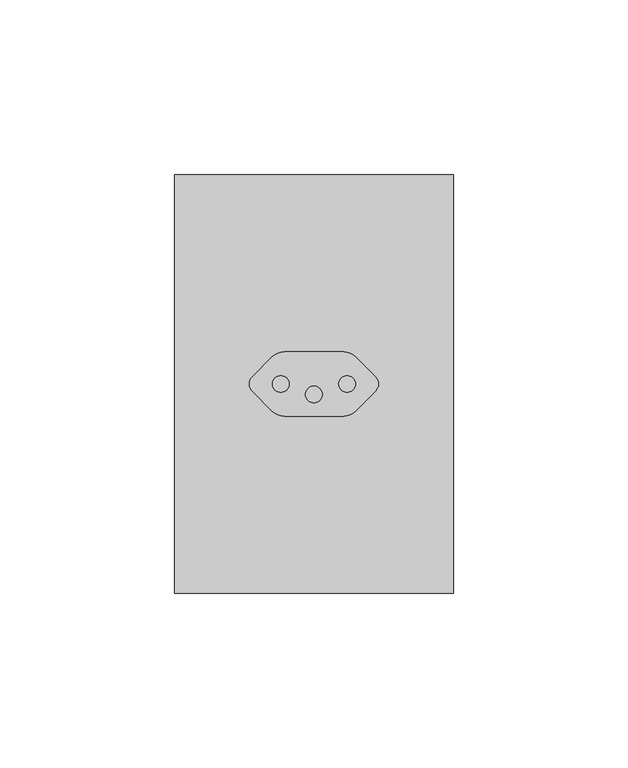
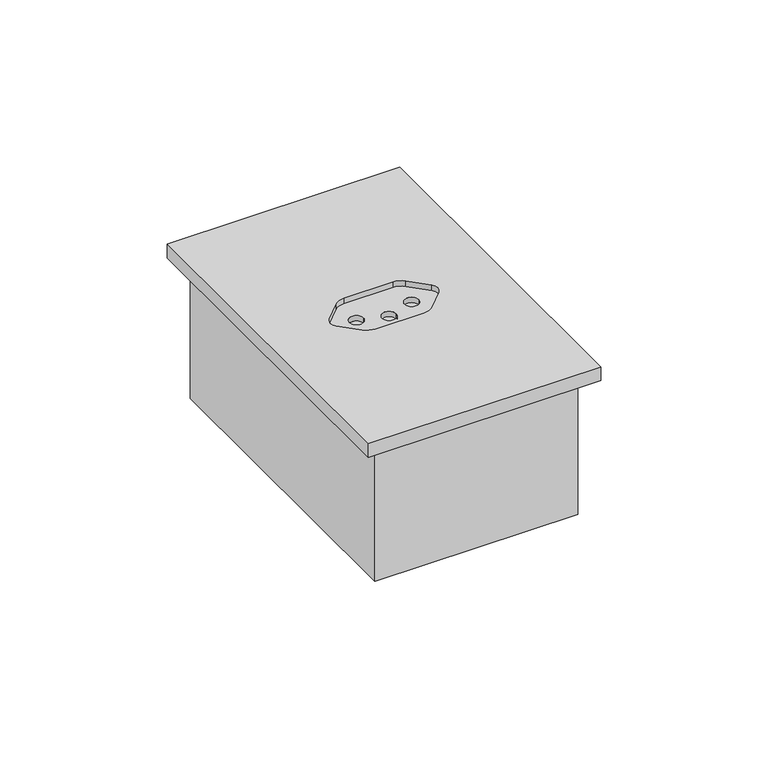
"""IFC4 building model written with IfcOpenShell, lengths in millimetres: proxy geometry, CAIXA VERTICE V7 : Tomada 20A 1s."""

from ifc_helpers import new_model, si_unit, frame, origin, place, context, project, spatial, polyline, circle_curve, faceted_brep, source, transform, mapped, element, save
from ifc_brep_helpers import plane_surface, revolved_surface, advanced_brep


def electrical_fixtures_8ee4f71d(model_context):
    return source(origin(), model_context, "Body", "SolidModel", [
        faceted_brep([(33.0, -2147.0, -48.0), (-33.0, -2147.0, -48.0), (-33.0, -2253.0, -48.0), (33.0, -2253.0, -48.0), (35.0, -2255.0, -50.0), (-35.0, -2255.0, -50.0), (-35.0, -2145.0, -50.0), (35.0, -2145.0, -50.0), (35.0, -2255.0, 0.0), (-35.0, -2255.0, 0.0), (-35.0, -2145.0, 0.0), (35.0, -2145.0, 0.0), (33.0, -2253.0, 0.0), (-33.0, -2253.0, 0.0), (-33.0, -2147.0, 0.0), (33.0, -2147.0, 0.0)], [[[0, 1, 2, 3]], [[4, 5, 6, 7]], [[4, 8, 9, 5]], [[9, 10, 6, 5]], [[10, 11, 7, 6]], [[11, 8, 4, 7]], [[8, 11, 10, 9], [12, 13, 14, 15]], [[15, 0, 3, 12]], [[14, 1, 0, 15]], [[13, 2, 1, 14]], [[12, 3, 2, 13]]]),
        advanced_brep(
        [(40.0, -2260.0, 5.0), (40.0, -2140.0, 5.0), (-40.0, -2140.0, 5.0), (-40.0, -2260.0, 5.0), (8.4215729, -2190.75, 5.0), (11.9571068, -2192.2144661, 5.0), (17.6213203, -2197.8786797, 5.0), (17.6213203, -2202.1213203, 5.0), (11.9571068, -2207.7855339, 5.0), (8.4215729, -2209.25, 5.0), (-8.4215729, -2209.25, 5.0), (-11.9571068, -2207.7855339, 5.0), (-17.6213203, -2202.1213203, 5.0), (-17.6213203, -2197.8786797, 5.0), (-11.9571068, -2192.2144661, 5.0), (-8.4215729, -2190.75, 5.0), (-40.0, -2260.0, 0.0), (-40.0, -2140.0, 0.0), (40.0, -2140.0, 0.0), (40.0, -2260.0, 0.0), (8.4215729, -2190.75, 3.0), (-8.4215729, -2190.75, 3.0), (-11.9571068, -2192.2144661, 3.0), (-17.6213203, -2197.8786797, 3.0), (-17.6213203, -2202.1213203, 3.0), (-11.9571068, -2207.7855339, 3.0), (-8.4215729, -2209.25, 3.0), (8.4215729, -2209.25, 3.0), (11.9571068, -2207.7855339, 3.0), (17.6213203, -2202.1213203, 3.0), (17.6213203, -2197.8786797, 3.0), (11.9571068, -2192.2144661, 3.0), (-7.1, -2200.0, 3.0), (-11.9, -2200.0, 3.0), (11.9, -2200.0, 3.0), (7.1, -2200.0, 3.0), (2.4, -2203.0, 3.0), (-2.4, -2203.0, 3.0), (-11.9, -2200.0, 1.0), (-7.1, -2200.0, 1.0), (7.1, -2200.0, 1.0), (11.9, -2200.0, 1.0), (-2.4, -2203.0, 1.0), (2.4, -2203.0, 1.0)],
        [
            (0, 1),
            (1, 2),
            (2, 3),
            (3, 0),
            (4, 5, circle_curve(frame((8.4215729, -2195.75, 5.0), z_axis=(0.0, 0.0, -1.0), x_axis=(-1.0, 0.0, 0.0)), 5.0)),
            (5, 6),
            (6, 7, circle_curve(frame((15.5, -2200.0, 5.0), z_axis=(0.0, 0.0, -1.0), x_axis=(-1.0, 0.0, 0.0)), 3.0)),
            (7, 8),
            (8, 9, circle_curve(frame((8.4215729, -2204.25, 5.0), z_axis=(0.0, 0.0, -1.0), x_axis=(-1.0, 0.0, 0.0)), 5.0)),
            (9, 10),
            (10, 11, circle_curve(frame((-8.4215729, -2204.25, 5.0), z_axis=(0.0, 0.0, -1.0), x_axis=(-1.0, 0.0, 0.0)), 5.0)),
            (11, 12),
            (12, 13, circle_curve(frame((-15.5, -2200.0, 5.0), z_axis=(0.0, 0.0, -1.0), x_axis=(-1.0, 0.0, 0.0)), 3.0)),
            (13, 14),
            (14, 15, circle_curve(frame((-8.4215729, -2195.75, 5.0), z_axis=(0.0, 0.0, -1.0), x_axis=(-1.0, 0.0, 0.0)), 5.0)),
            (15, 4),
            (16, 17),
            (17, 18),
            (18, 19),
            (19, 16),
            (3, 16),
            (19, 0),
            (2, 17),
            (1, 18),
            (20, 21),
            (21, 22, circle_curve(frame((-8.4215729, -2195.75, 3.0), z_axis=(0.0, 0.0, 1.0), x_axis=(-1.0, 0.0, 0.0)), 5.0)),
            (22, 23),
            (23, 24, circle_curve(frame((-15.5, -2200.0, 3.0), z_axis=(0.0, 0.0, 1.0), x_axis=(-1.0, 0.0, 0.0)), 3.0)),
            (24, 25),
            (25, 26, circle_curve(frame((-8.4215729, -2204.25, 3.0), z_axis=(0.0, 0.0, 1.0), x_axis=(-1.0, 0.0, 0.0)), 5.0)),
            (26, 27),
            (27, 28, circle_curve(frame((8.4215729, -2204.25, 3.0), z_axis=(0.0, 0.0, 1.0), x_axis=(-1.0, 0.0, 0.0)), 5.0)),
            (28, 29),
            (29, 30, circle_curve(frame((15.5, -2200.0, 3.0), z_axis=(0.0, 0.0, 1.0), x_axis=(-1.0, 0.0, 0.0)), 3.0)),
            (30, 31),
            (31, 20, circle_curve(frame((8.4215729, -2195.75, 3.0), z_axis=(0.0, 0.0, 1.0), x_axis=(-1.0, 0.0, 0.0)), 5.0)),
            (32, 33, circle_curve(frame((-9.5, -2200.0, 3.0), z_axis=(0.0, 0.0, -1.0), x_axis=(1.0, -2.301812013077709e-12, 0.0)), 2.4)),
            (33, 32, circle_curve(frame((-9.5, -2200.0, 3.0), z_axis=(0.0, 0.0, -1.0), x_axis=(1.0, -2.301812013077709e-12, 0.0)), 2.4)),
            (34, 35, circle_curve(frame((9.5, -2200.0, 3.0), z_axis=(0.0, 0.0, -1.0), x_axis=(1.0, -2.301812013077709e-12, 0.0)), 2.4)),
            (35, 34, circle_curve(frame((9.5, -2200.0, 3.0), z_axis=(0.0, 0.0, -1.0), x_axis=(1.0, -2.301812013077709e-12, 0.0)), 2.4)),
            (36, 37, circle_curve(frame((0.0, -2203.0, 3.0), z_axis=(0.0, 0.0, -1.0), x_axis=(1.0, -2.301812013077709e-12, 0.0)), 2.4)),
            (37, 36, circle_curve(frame((0.0, -2203.0, 3.0), z_axis=(0.0, 0.0, -1.0), x_axis=(1.0, -2.301812013077709e-12, 0.0)), 2.4)),
            (20, 4),
            (15, 21),
            (14, 22),
            (13, 23),
            (12, 24),
            (11, 25),
            (10, 26),
            (9, 27),
            (8, 28),
            (7, 29),
            (6, 30),
            (5, 31),
            (38, 39, circle_curve(frame((-9.5, -2200.0, 1.0), z_axis=(0.0, 0.0, 1.0), x_axis=(1.0, -2.301812013077709e-12, 0.0)), 2.4)),
            (39, 38, circle_curve(frame((-9.5, -2200.0, 1.0), z_axis=(0.0, 0.0, 1.0), x_axis=(1.0, -2.301812013077709e-12, 0.0)), 2.4)),
            (40, 41, circle_curve(frame((9.5, -2200.0, 1.0), z_axis=(0.0, 0.0, 1.0), x_axis=(1.0, -2.301812013077709e-12, 0.0)), 2.4)),
            (41, 40, circle_curve(frame((9.5, -2200.0, 1.0), z_axis=(0.0, 0.0, 1.0), x_axis=(1.0, -2.301812013077709e-12, 0.0)), 2.4)),
            (42, 43, circle_curve(frame((0.0, -2203.0, 1.0), z_axis=(0.0, 0.0, 1.0), x_axis=(1.0, -2.301812013077709e-12, 0.0)), 2.4)),
            (43, 42, circle_curve(frame((0.0, -2203.0, 1.0), z_axis=(0.0, 0.0, 1.0), x_axis=(1.0, -2.301812013077709e-12, 0.0)), 2.4)),
            (33, 38),
            (39, 32),
            (35, 40),
            (41, 34),
            (37, 42),
            (43, 36),
        ],
        [
            plane_surface(frame((-60.0, -2260.0, 5.0), z_axis=(0.0, 0.0, 1.0), x_axis=(-1.0, 0.0, 0.0))),
            plane_surface(frame((-60.0, -2260.0, 0.0), z_axis=(0.0, 0.0, -1.0), x_axis=(1.0, 0.0, 0.0))),
            plane_surface(frame((40.0, -2260.0, 5.0), z_axis=(0.0, -1.0, 0.0), x_axis=(0.0, 0.0, -1.0))),
            plane_surface(frame((-40.0, -2260.0, 5.0), z_axis=(-1.0, 0.0, 0.0), x_axis=(0.0, 0.0, -1.0))),
            plane_surface(frame((-40.0, -2140.0, 5.0), z_axis=(0.0, 1.0, 0.0), x_axis=(0.0, 0.0, -1.0))),
            plane_surface(frame((40.0, -2140.0, 5.0), z_axis=(1.0, 0.0, 0.0), x_axis=(0.0, 0.0, -1.0))),
            plane_surface(frame((3.4215729, -2195.75, 3.0), z_axis=(0.0, 0.0, 1.0), x_axis=(0.0, -1.0, 0.0))),
            plane_surface(frame((-8.4215729, -2190.75, 5.0), z_axis=(0.0, -1.0, 0.0), x_axis=(0.0, 0.0, -1.0))),
            revolved_surface(polyline([(-13.4215729, -2195.75, 5.0), (-13.4215729, -2195.75, 3.0)]), (-8.4215729, -2195.75, 3.0), (0.0, 0.0, 1.0)),
            plane_surface(frame((-17.6213203, -2197.8786797, 5.0), z_axis=(0.7071067811865045, -0.7071067811865905, 0.0), x_axis=(0.0, 0.0, -1.0))),
            revolved_surface(polyline([(-18.5, -2200.0, 5.0), (-18.5, -2200.0, 3.0)]), (-15.5, -2200.0, 3.0), (0.0, 0.0, 1.0)),
            plane_surface(frame((-11.9571068, -2207.7855339, 5.0), z_axis=(0.7071067811865515, 0.7071067811865437, 0.0), x_axis=(0.0, 0.0, -1.0))),
            revolved_surface(polyline([(-13.4215729, -2204.25, 5.0), (-13.4215729, -2204.25, 3.0)]), (-8.4215729, -2204.25, 3.0), (0.0, 0.0, 1.0)),
            plane_surface(frame((8.4215729, -2209.25, 5.0), z_axis=(0.0, 1.0, 0.0), x_axis=(0.0, 0.0, -1.0))),
            revolved_surface(polyline([(3.4215728999999993, -2204.25, 5.0), (3.4215728999999993, -2204.25, 3.0)]), (8.4215729, -2204.25, 3.0), (0.0, 0.0, 1.0)),
            plane_surface(frame((17.6213203, -2202.1213203, 5.0), z_axis=(-0.7071067811865307, 0.7071067811865643, 0.0), x_axis=(0.0, 0.0, -1.0))),
            revolved_surface(polyline([(12.5, -2200.0, 5.0), (12.5, -2200.0, 3.0)]), (15.5, -2200.0, 3.0), (0.0, 0.0, 1.0)),
            plane_surface(frame((11.9571068, -2192.2144661, 5.0), z_axis=(-0.7071067811865893, -0.7071067811865058, 0.0), x_axis=(0.0, 0.0, -1.0))),
            revolved_surface(polyline([(3.4215728999999993, -2195.75, 5.0), (3.4215728999999993, -2195.75, 3.0)]), (8.4215729, -2195.75, 3.0), (0.0, 0.0, 1.0)),
            plane_surface(frame((-7.1, -2200.0, 1.0), z_axis=(0.0, 0.0, 1.0), x_axis=(2.301812013077709e-12, 1.0, 0.0))),
            revolved_surface(polyline([(-7.1, -2200.0000000000055, 3.0), (-7.1, -2200.0000000000055, 1.0)]), (-9.5, -2200.0, 1.0), (0.0, 0.0, 1.0)),
            revolved_surface(polyline([(11.9, -2200.0000000000055, 3.0), (11.9, -2200.0000000000055, 1.0)]), (9.5, -2200.0, 5.0), (0.0, 0.0, 1.0)),
            revolved_surface(polyline([(2.4, -2203.0000000000055, 3.0), (2.4, -2203.0000000000055, 1.0)]), (0.0, -2203.0, 5.0), (0.0, 0.0, 1.0)),
        ],
        [
            (0, [[1, 2, 3, 4], [5, 6, 7, 8, 9, 10, 11, 12, 13, 14, 15, 16]]),
            (1, [[17, 18, 19, 20]]),
            (2, [[21, -20, 22, -4]]),
            (3, [[23, -17, -21, -3]]),
            (4, [[24, -18, -23, -2]]),
            (5, [[-22, -19, -24, -1]]),
            (6, [[25, 26, 27, 28, 29, 30, 31, 32, 33, 34, 35, 36], [37, 38], [39, 40], [41, 42]]),
            (7, [[43, -16, 44, -25]]),
            (8, [[-44, -15, 45, -26]]),
            (9, [[-45, -14, 46, -27]]),
            (10, [[-46, -13, 47, -28]]),
            (11, [[-47, -12, 48, -29]]),
            (12, [[-48, -11, 49, -30]]),
            (13, [[-49, -10, 50, -31]]),
            (14, [[-50, -9, 51, -32]]),
            (15, [[-51, -8, 52, -33]]),
            (16, [[-52, -7, 53, -34]]),
            (17, [[-53, -6, 54, -35]]),
            (18, [[-54, -5, -43, -36]]),
            (19, [[55, 56]]),
            (19, [[57, 58]]),
            (19, [[59, 60]]),
            (20, [[61, -56, 62, -38]]),
            (20, [[-62, -55, -61, -37]]),
            (21, [[63, -58, 64, -40]]),
            (21, [[-64, -57, -63, -39]]),
            (22, [[65, -60, 66, -42]]),
            (22, [[-66, -59, -65, -41]]),
        ],
    ),
    ])


if __name__ == "__main__":
    model = new_model("IFC4")
    model_context = context("Model", 3, world=origin())
    ifc_project = project(units=[si_unit("LENGTHUNIT", "METRE", prefix="MILLI")], contexts=[model_context])
    site = spatial("IfcSite", under=ifc_project)
    building = spatial("IfcBuilding", under=site)
    placement = place(None, origin())
    electrical_fixtures_shape = electrical_fixtures_8ee4f71d(model_context)
    element("IfcBuildingElementProxy", 1, Name="CAIXA VERTICE V7 : Tomada 20A 1s", ObjectType="CAIXA VERTICE V7 : Tomada 20A 1s", at=placement, inside=building, context=model_context, shape_type="MappedRepresentation", body=[
        mapped(electrical_fixtures_shape, transform((0.0, 0.0, 0.0), x_axis=(1.0, 0.0, 0.0), y_axis=(0.0, 1.0, 0.0), z_axis=(0.0, 0.0, 1.0))),
    ])
    save(model, "model.ifc")

# Revit data of these elements
# Type "CAIXA VERTICE V7 : Tomada 20A 1s"
#   URL = "www.facebook.com/verticetreinamentos"
#   SEÇÃO [instance default] = ""
#   Rotação [instance default] = 0.00°
#   LARGURA DA TAMPA = 0.08 m
#   BORDA = 0.01 m
#   ALTURA DE INSTALAÇÃO [instance default] = 1.10 m
#   Distância Anotação [instance default] = 0.0015 m
#   ALTURA DA TAMPA = 0.12 m
#   Vertical [instance default] = yes
#   VER SEÇÃO [instance default] = no
#   SHADE ESQ [instance default] = no
#   SHADE DIR [instance default] = yes
#   HORIZONTAL [instance default] = no
#   ANDAR COM A LEGENDA [instance default] = 0
#   Material Tampa [instance default] = Plástico, branco opaco
#   Caixa = element 1798517
#   Anotação = element 1798531
#   Default Elevation = 0
# Element 1 (IfcBuildingElementProxy, "CAIXA VERTICE V7 : Tomada 20A 1s")
#   ALTURA DE INSTALAÇÃO = 2.20 m
#   SHADE ESQ = yes
#   Materials on its faces: "Plástico, branco opaco"
# Materials
#   "Plástico, branco opaco": class "Plástico", colour RGB 120 120 120, transparency 0, Description = "Plastic, generic, opaque white", Cost = 0
